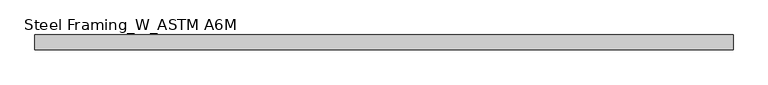
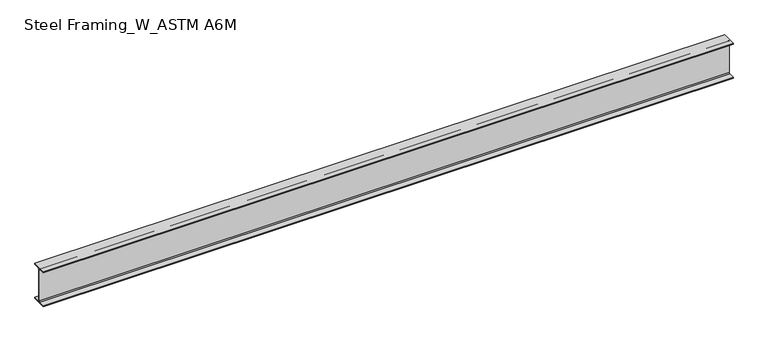
"""IFC4 building model written with IfcOpenShell, lengths in millimetres: beam geometry, Steel Framing_W_ASTM A6M : H_SB_AR_S02_W530x101_RB1."""

from ifc_helpers import new_model, si_unit, point, frame, frame_2d, origin, place, context, project, spatial, polyline, circle_curve, trimmed, segment, composite_curve, outline, extrude, source, transform, mapped, element, save


def steel_framing_w_astm_a6m_b3a50ba3(model_context):
    return source(origin(), model_context, "Body", "SweptSolid", [
        extrude(outline(composite_curve([segment(polyline([(105.0, -250.6), (105.0, -268.0), (-105.0, -268.0), (-105.0, -250.6), (-18.25, -250.6)]), True, "CONTINUOUS"), segment(trimmed(circle_curve(frame_2d((-18.25, -237.8)), 12.8), [point((-18.25, -250.6))], [point((-5.45, -237.8))], True, "CARTESIAN"), True, "CONTINUOUS"), segment(polyline([(-5.45, -237.8), (-5.45, 237.8)]), True, "CONTINUOUS"), segment(trimmed(circle_curve(frame_2d((-18.25, 237.8)), 12.8), [point((-5.45, 237.8))], [point((-18.25, 250.6))], True, "CARTESIAN"), True, "CONTINUOUS"), segment(polyline([(-18.25, 250.6), (-105.0, 250.6), (-105.0, 268.0), (105.0, 268.0), (105.0, 250.6), (18.25, 250.6)]), True, "CONTINUOUS"), segment(trimmed(circle_curve(frame_2d((18.25, 237.8)), 12.8), [point((18.25, 250.6))], [point((5.45, 237.8))], True, "CARTESIAN"), True, "CONTINUOUS"), segment(polyline([(5.45, 237.8), (5.45, -237.8)]), True, "CONTINUOUS"), segment(trimmed(circle_curve(frame_2d((18.25, -237.8)), 12.8), [point((5.45, -237.8))], [point((18.25, -250.6))], True, "CARTESIAN"), True, "CONTINUOUS"), segment(polyline([(18.25, -250.6), (105.0, -250.6)]), True, "CONTINUOUS")], self_intersect=False)), frame((-4987.2, 0.0, 0.0), z_axis=(1.0, 0.0, 0.0), x_axis=(0.0, 1.0, 0.0)), (0.0, 0.0, 1.0), 9987.2),
    ])


if __name__ == "__main__":
    model = new_model("IFC4")
    model_context = context("Model", 3, world=origin())
    ifc_project = project(units=[si_unit("LENGTHUNIT", "METRE", prefix="MILLI")], contexts=[model_context])
    site = spatial("IfcSite", under=ifc_project)
    building = spatial("IfcBuilding", under=site)
    placement = place(None, origin())
    steel_framing_w_astm_a6m_shape = steel_framing_w_astm_a6m_b3a50ba3(model_context)
    element("IfcBeam", 1, ObjectType="Steel Framing_W_ASTM A6M : H_SB_AR_S02_W530x101_RB1", at=placement, inside=building, context=model_context, shape_type="MappedRepresentation", body=[
        mapped(steel_framing_w_astm_a6m_shape, transform((0.0, 0.0, 0.0), x_axis=(1.0, 0.0, 0.0), y_axis=(0.0, 1.0, 0.0), z_axis=(0.0, 0.0, 1.0))),
    ])
    save(model, "model.ifc")

# Revit data of these elements
# Type "Steel Framing_W_ASTM A6M : H_SB_AR_S02_W530x101_RB1"
#   Type Mark = "RB1"
#   Section Name Key = "W21x68"
#   Width = 21.0 cm
#   Web Thickness = 1.09 cm
#   Web Fillet = 1.28 cm
#   Warping Constant = 1820000.0 cm⁶
#   Torsional Moment of Inertia = 102.00 cm⁴
#   Section Area = 129.0 cm²
#   Plastic Modulus weak axis = 400.0 cm³
#   Plastic Modulus strong axis = 2620.0 cm³
#   Perimeter = 1.87 m²/m
#   Nominal Weight = 101.00 kgf/m
#   Moment of Inertia weak axis = 2690.00 cm⁴
#   Moment of Inertia strong axis = 61600.00 cm⁴
#   Height = 53.6 cm
#   Flange Thickness = 1.74 cm
#   Elastic Modulus weak axis = 257.0 cm³
#   Elastic Modulus strong axis = 2290.0 cm³
#   Centroid Vertical = 26.8 cm
#   Centroid Horizontal = 10.5 cm
#   Length [instance default] = 1500 mm
#   Structural Material [instance default] = Steel, 45-345
#   Bolt Spacing = 0
#   Assembly Code = ""
# Element 1 (IfcBeam, "Steel Framing_W_ASTM A6M : H_SB_AR_S02_W530x101_RB1")
#   Materials on its faces: "Steel, 45-345"
# Materials
#   "Steel, 45-345": class "Metal", colour RGB 189 187 185, transparency 0, Description = "Steel 345 MPa", Cost = 0
